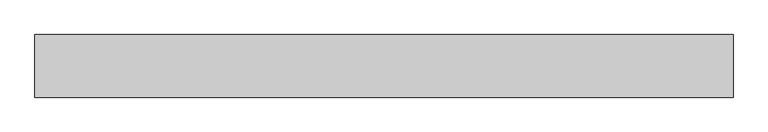
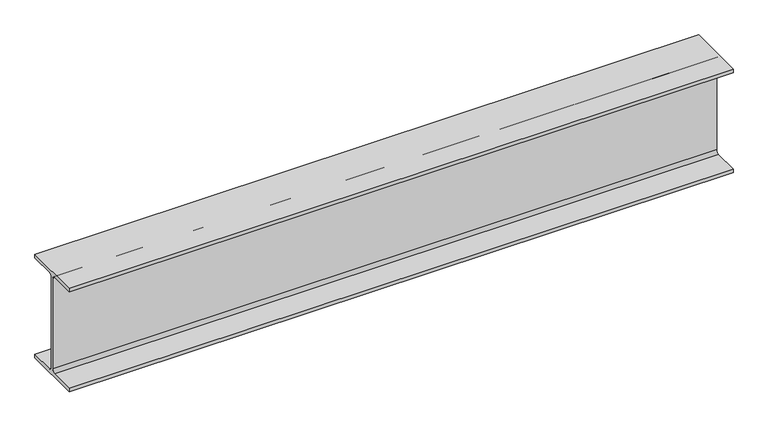
"""IFC4 building model written with IfcOpenShell, lengths in millimetres: beam geometry, Steel Beam_H-KSD3502 : H_SB_ASB_H-194x150x6x9."""

from ifc_helpers import new_model, si_unit, point, frame, frame_2d, origin, place, context, project, spatial, polyline, circle_curve, trimmed, segment, composite_curve, outline, extrude, source, transform, mapped, element, save


def beam_91d8de06(model_context):
    return source(origin(), model_context, "Body", "SweptSolid", [
        extrude(outline(composite_curve([segment(polyline([(-82.5, -141.5), (-11.9, -141.5)]), True, "CONTINUOUS"), segment(trimmed(circle_curve(frame_2d((-11.9, -132.6)), 8.9), [point((-11.9, -141.5))], [point((-3.0, -132.6))], True, "CARTESIAN"), True, "CONTINUOUS"), segment(polyline([(-3.0, -132.6), (-3.0, 132.6)]), True, "CONTINUOUS"), segment(trimmed(circle_curve(frame_2d((-11.9, 132.6)), 8.9), [point((-3.0, 132.6))], [point((-11.9, 141.5))], True, "CARTESIAN"), True, "CONTINUOUS"), segment(polyline([(-11.9, 141.5), (-82.5, 141.5), (-82.5, 151.7), (82.5, 151.7), (82.5, 141.5), (11.9, 141.5)]), True, "CONTINUOUS"), segment(trimmed(circle_curve(frame_2d((11.9, 132.6)), 8.9), [point((11.9, 141.5))], [point((3.0, 132.6))], True, "CARTESIAN"), True, "CONTINUOUS"), segment(polyline([(3.0, 132.6), (3.0, -132.6)]), True, "CONTINUOUS"), segment(trimmed(circle_curve(frame_2d((11.9, -132.6)), 8.9), [point((3.0, -132.6))], [point((11.9, -141.5))], True, "CARTESIAN"), True, "CONTINUOUS"), segment(polyline([(11.9, -141.5), (82.5, -141.5), (82.5, -151.7), (-82.5, -151.7), (-82.5, -141.5)]), True, "CONTINUOUS")], self_intersect=False)), frame((-851.3274068, 0.0, 0.0), z_axis=(1.0, 0.0, 0.0), x_axis=(0.0, 1.0, 0.0)), (0.0, 0.0, 1.0), 1839.6820153),
    ])


if __name__ == "__main__":
    model = new_model("IFC4")
    model_context = context("Model", 3, world=origin())
    ifc_project = project(units=[si_unit("LENGTHUNIT", "METRE", prefix="MILLI")], contexts=[model_context])
    site = spatial("IfcSite", under=ifc_project)
    building = spatial("IfcBuilding", under=site)
    placement = place(None, origin())
    beam_shape = beam_91d8de06(model_context)
    element("IfcBeam", 1, ObjectType="Steel Beam_H-KSD3502 : H_SB_ASB_H-194x150x6x9", at=placement, inside=building, context=model_context, shape_type="MappedRepresentation", body=[
        mapped(beam_shape, transform((0.0, 0.0, 0.0), x_axis=(1.0, 0.0, 0.0), y_axis=(0.0, 1.0, 0.0), z_axis=(0.0, 0.0, 1.0))),
    ])
    save(model, "model.ifc")

# Revit data of these elements
# Type "Steel Beam_H-KSD3502 : H_SB_ASB_H-194x150x6x9"
#   Width = 15.0 cm
#   Web Thickness = 0.6 cm
#   Web Fillet = 1.3 cm
#   Warping Constant = 43316.0 cm⁶
#   Torsional Moment of Inertia = 8.622 cm⁴
#   Torsional Modulus = 1.0 cm³
#   Section Area = 39.01 cm²
#   Plastic Modulus weak axis = 104.0 cm³
#   Plastic Modulus strong axis = 309.0 cm³
#   Perimeter = 0.95 m²/m
#   Nominal Weight = 30.60 kgf/m
#   Moment of Inertia weak axis = 507.00 cm⁴
#   Moment of Inertia strong axis = 2690.00 cm⁴
#   Height = 19.4 cm
#   Flange Thickness = 0.9 cm
#   Elastic Modulus weak axis = 67.6 cm³
#   Elastic Modulus strong axis = 277.0 cm³
#   Centroid Vertical = 9.7 cm
#   Centroid Horizontal = 7.5 cm
#   Length [instance default] = 1.5240 m
#   Structural Material [instance default] = Steel, 45-345
#   Assembly Code = ""
# Element 1 (IfcBeam, "Steel Beam_H-KSD3502 : H_SB_ASB_H-194x150x6x9")
#   Structural Material = none
# Materials
#   "Steel, 45-345": class "Metal", colour RGB 189 187 185, transparency 0, Description = "Steel 345 MPa", Cost = 0
